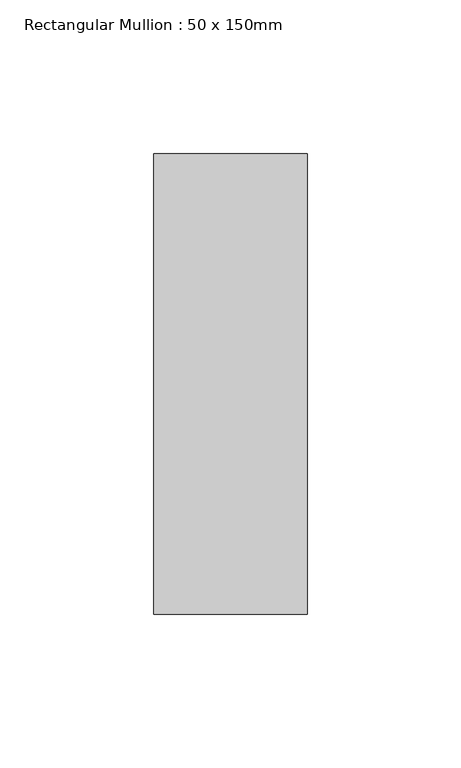
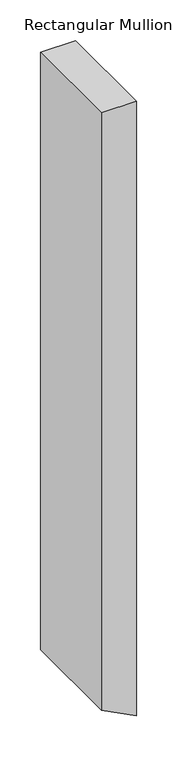
"""IFC4 building model written with IfcOpenShell, lengths in millimetres: member geometry, Rectangular Mullion : 50 x 150mm."""

from ifc_helpers import new_model, si_unit, frame, origin, place, context, project, spatial, polyline, outline, extrude, source, transform, mapped, element, save


def rectangular_mullion_50_x_150mm_79f3c384(model_context):
    return source(origin(), model_context, "Body", "SweptSolid", [
        extrude(outline(polyline([(0.0, 0.0), (0.0, -50.0), (-897.962266, -50.0), (-923.9906185, 0.0), (0.0, 0.0)])), frame((0.0, -75.0, 0.0), z_axis=(0.0, 1.0, 0.0), x_axis=(0.0, 0.0, 1.0)), (0.0, 0.0, 1.0), 150.0),
    ])


if __name__ == "__main__":
    model = new_model("IFC4")
    model_context = context("Model", 3, world=origin())
    ifc_project = project(units=[si_unit("LENGTHUNIT", "METRE", prefix="MILLI")], contexts=[model_context])
    site = spatial("IfcSite", under=ifc_project)
    building = spatial("IfcBuilding", under=site)
    placement = place(None, origin())
    rectangular_mullion_50_x_150mm_shape = rectangular_mullion_50_x_150mm_79f3c384(model_context)
    element("IfcMember", 1, ObjectType="Rectangular Mullion : 50 x 150mm", at=placement, inside=building, context=model_context, shape_type="MappedRepresentation", body=[
        mapped(rectangular_mullion_50_x_150mm_shape, transform((0.0, 0.0, 0.0), x_axis=(1.0, 0.0, 0.0), y_axis=(0.0, 1.0, 0.0), z_axis=(0.0, 0.0, 1.0))),
    ])
    save(model, "model.ifc")

# Revit data of these elements
# Type "Rectangular Mullion : 50 x 150mm"
#   built-in parameter 1007304 = 0.492126 (stored number, unit not read)
#   built-in parameter 1007301 = 0.082021 (stored number, unit not read)
#   built-in parameter 1007300 = 0.082021 (stored number, unit not read)
# Element 1 (IfcMember, "Rectangular Mullion : 50 x 150mm")
#   Materials on its faces: "Aluminium"
# Materials
#   "Aluminium": class "Metal", colour RGB 247 247 247, transparency 0, Description = "Aluminium 6061", Cost = 0
